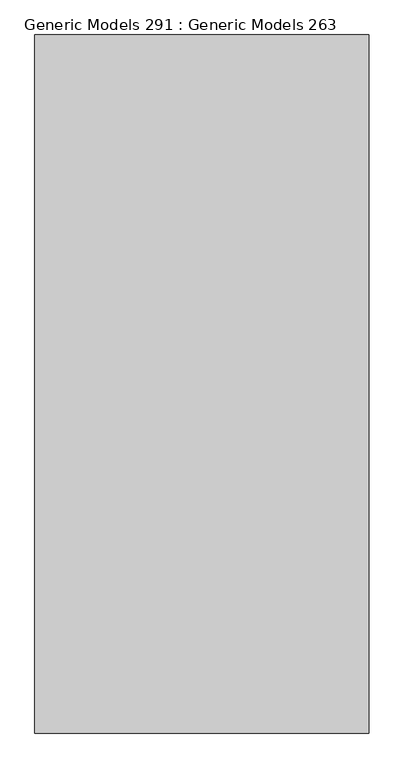
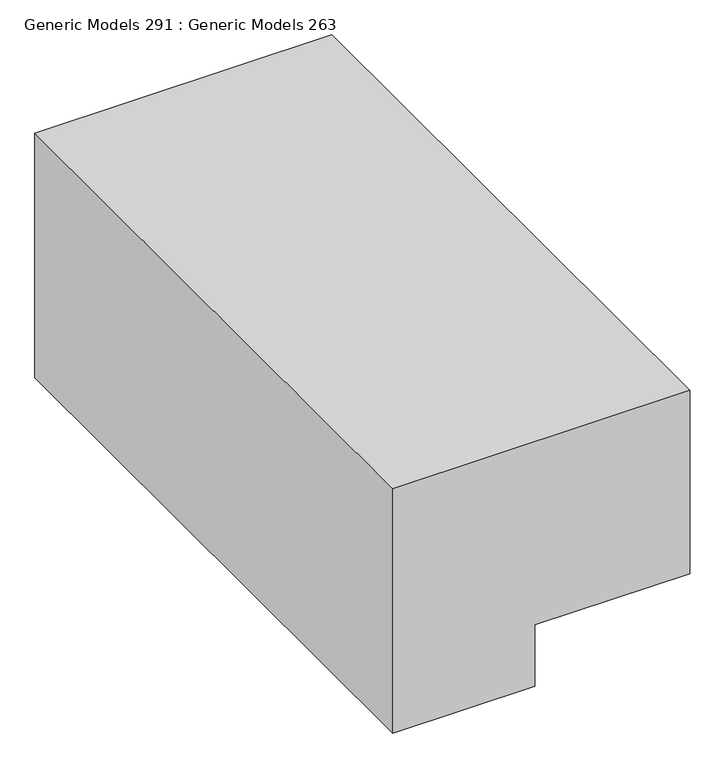
"""IFC4 building model written with IfcOpenShell, lengths in millimetres: proxy geometry, Generic Models 291 : Generic Models 263."""

from ifc_helpers import new_model, si_unit, frame, origin, place, context, project, spatial, polyline, outline, extrude, source, transform, mapped, element, save


def generic_models_291_generic_models_263_452afd1b(model_context):
    return source(origin(), model_context, "Body", "SweptSolid", [
        extrude(outline(polyline([(-381.0, 62319.1797726), (0.0, 62319.1797726), (0.0, 61734.9797726), (-508.0, 61734.9797726), (-508.0, 62014.3797726), (-381.0, 62014.3797726), (-381.0, 62319.1797726)])), frame((0.0, -94.4486541, 0.0), z_axis=(0.0, 1.0, 0.0), x_axis=(0.0, 0.0, 1.0)), (0.0, 0.0, 1.0), 1219.2),
    ])


if __name__ == "__main__":
    model = new_model("IFC4")
    model_context = context("Model", 3, world=origin())
    ifc_project = project(units=[si_unit("LENGTHUNIT", "METRE", prefix="MILLI")], contexts=[model_context])
    site = spatial("IfcSite", under=ifc_project)
    building = spatial("IfcBuilding", under=site)
    placement = place(None, origin())
    generic_models_291_generic_models_263_shape = generic_models_291_generic_models_263_452afd1b(model_context)
    element("IfcBuildingElementProxy", 1, Name="Generic Models 291 : Generic Models 263", ObjectType="Generic Models 291 : Generic Models 263", at=placement, inside=building, context=model_context, shape_type="MappedRepresentation", body=[
        mapped(generic_models_291_generic_models_263_shape, transform((0.0, 0.0, 0.0), x_axis=(1.0, 0.0, 0.0), y_axis=(0.0, 1.0, 0.0), z_axis=(0.0, 0.0, 1.0))),
    ])
    save(model, "model.ifc")

# Revit data of these elements
# Element 1 (IfcBuildingElementProxy, "Generic Models 291 : Generic Models 263")
#   Materials on its faces: "GRADED BACKFILL"
# Materials
#   "GRADED BACKFILL": class "Miscellaneous", colour RGB 128 97 77, transparency 0, Cost = 0
